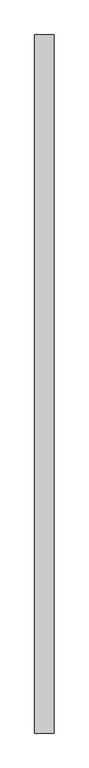
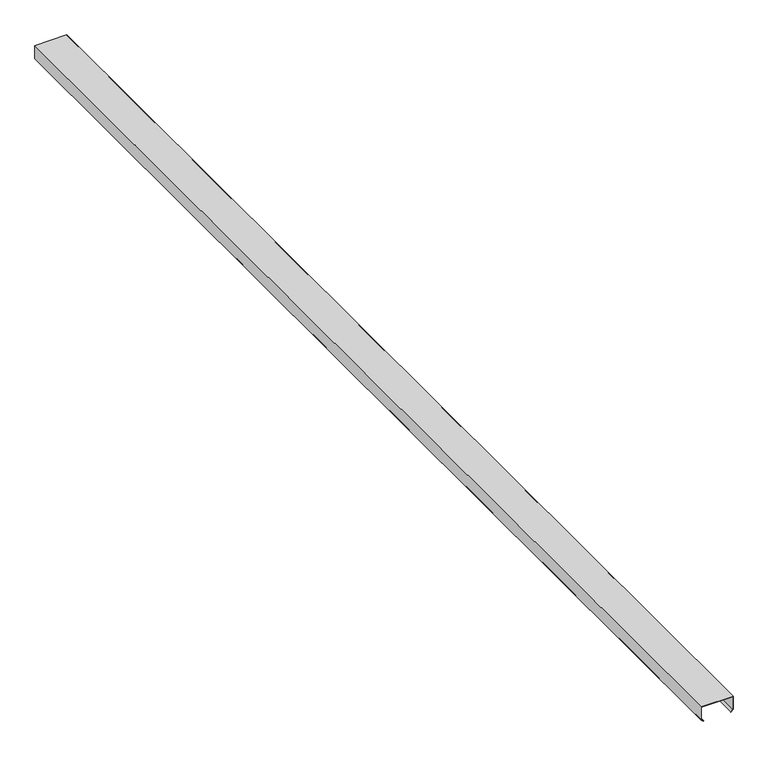
"""IFC4 building model written with IfcOpenShell, lengths in millimetres: proxy geometry, Generic Models 7:Generic Models 1:1:Generic Models 1:1 : Generic Models 7:Generic Models 1:337419:19 : Generic Models 7:Generic Models 1:1:Generic Models 1:1 : Generic Models 7:Generic Models 1:337419:306201."""

import ifcopenshell
import ifcopenshell.guid

model = None  # the IFC model being written
_history = None  # IfcOwnerHistory: only IFC2X3 demands one
_inside = {}  # id of a spatial element -> (the spatial element, [elements in it])
_under = {}  # id of a project, library or spatial element -> (it, [spatial elements below it])
_declared = {}  # id of a project -> (the project, [libraries it declares])
_typed = {}  # id of a type object -> (the type object, [elements of that type])
_made_of = {}  # id of a material, layer set ... -> (it, [elements and type objects made of it])


def new_model(schema):
    """Start an empty IFC model of exactly this schema.

    Asked for "IFC4X3", IfcOpenShell would pick the latest addendum, in which some entities
    have other attributes; the version numbers below select the first issue.
    IFC2X3 requires an IfcOwnerHistory on every rooted entity: one is made here for all.
    """
    global model, _history
    if schema == "IFC4X3":
        model = ifcopenshell.file(schema_version=(4, 3, 0, 0))
    else:
        model = ifcopenshell.file(schema=schema)
    _inside.clear()
    _under.clear()
    _declared.clear()
    _typed.clear()
    _made_of.clear()
    _history = None
    if model.schema == "IFC2X3":
        org = make("IfcOrganization", Name="unknown")
        user = make(
            "IfcPersonAndOrganization",
            ThePerson=make("IfcPerson", FamilyName="unknown"),
            TheOrganization=org,
        )
        app = make(
            "IfcApplication",
            ApplicationDeveloper=org,
            Version="unknown",
            ApplicationFullName="unknown",
            ApplicationIdentifier="unknown",
        )
        _history = make(
            "IfcOwnerHistory",
            OwningUser=user,
            OwningApplication=app,
            ChangeAction="ADDED",
            CreationDate=0,
        )
    return model


def make(cls, **values):
    """One entity of the class cls with the attributes given. An attribute that is None is left unset."""
    return model.create_entity(
        cls, **{name: value for name, value in values.items() if value is not None}
    )


def rooted(cls, **values):
    """An entity with a GlobalId (a new one), such as an element, a storey or a relation."""
    return make(cls, GlobalId=ifcopenshell.guid.new(), OwnerHistory=_history, **values)


def si_unit(unit_type, name, prefix=None):
    """IfcSIUnit, for example si_unit("LENGTHUNIT", "METRE", prefix="MILLI")."""
    return make("IfcSIUnit", UnitType=unit_type, Prefix=prefix, Name=name)


def assignment(units):
    """IfcUnitAssignment: the units of a project."""
    return None if units is None else make("IfcUnitAssignment", Units=units)


def point(xyz):
    """IfcCartesianPoint."""
    return None if xyz is None else make("IfcCartesianPoint", Coordinates=xyz)


def direction(xyz):
    """IfcDirection."""
    return None if xyz is None else make("IfcDirection", DirectionRatios=xyz)


def frame(location, z_axis=None, x_axis=None):
    """IfcAxis2Placement3D, a coordinate frame: its origin and axes. An axis left out is left unset."""
    return make(
        "IfcAxis2Placement3D",
        Location=point(location),
        Axis=direction(z_axis),
        RefDirection=direction(x_axis),
    )


def origin():
    """The frame at (0, 0, 0) with its axes left unset."""
    return frame((0.0, 0.0, 0.0))


def place(relative_to, where):
    """IfcLocalPlacement: puts the frame where relative to a parent placement (None: the world)."""
    return make(
        "IfcLocalPlacement", PlacementRelTo=relative_to, RelativePlacement=where
    )


def context(
    kind, dimensions, precision=None, world=None, true_north=None, identifier=None
):
    """IfcGeometricRepresentationContext, for example the 3D "Model" context."""
    return make(
        "IfcGeometricRepresentationContext",
        ContextIdentifier=identifier,
        ContextType=kind,
        CoordinateSpaceDimension=dimensions,
        Precision=precision,
        WorldCoordinateSystem=world,
        TrueNorth=true_north,
    )


def project(units=None, contexts=None):
    """IfcProject with its units and contexts."""
    return rooted(
        "IfcProject",
        Name="project",
        RepresentationContexts=contexts,
        UnitsInContext=assignment(units),
    )


def spatial(cls, under=None, at=None, **own):
    """A site, building, storey or space (cls), placed at a placement, below another one or the project."""
    s = rooted(cls, ObjectPlacement=at, **own)
    if under is not None:
        _under.setdefault(under.id(), (under, []))[1].append(s)
    return s


def polyline(points):
    """IfcPolyline through the points."""
    return make("IfcPolyline", Points=[point(p) for p in points])


def outline(outer, holes=None, kind="AREA"):
    """IfcArbitraryClosedProfileDef: a profile drawn as a closed curve; with holes, ...WithVoids."""
    if holes is None:
        return make("IfcArbitraryClosedProfileDef", ProfileType=kind, OuterCurve=outer)
    return make(
        "IfcArbitraryProfileDefWithVoids",
        ProfileType=kind,
        OuterCurve=outer,
        InnerCurves=holes,
    )


def extrude(swept, where, along, depth):
    """IfcExtrudedAreaSolid: the profile swept, set in the frame where, extruded along a direction by depth."""
    return make(
        "IfcExtrudedAreaSolid",
        SweptArea=swept,
        Position=where,
        ExtrudedDirection=direction(along),
        Depth=depth,
    )


def shape(context_of_items, identifier, shape_type, items):
    """IfcShapeRepresentation: the items that make up one representation, for example the "Body"."""
    return make(
        "IfcShapeRepresentation",
        ContextOfItems=context_of_items,
        RepresentationIdentifier=identifier,
        RepresentationType=shape_type,
        Items=items,
    )


def source(mapping_origin, context_of_items, identifier, shape_type, items):
    """IfcRepresentationMap: a shape defined once, which mapped items show again and again."""
    return make(
        "IfcRepresentationMap",
        MappingOrigin=mapping_origin,
        MappedRepresentation=shape(context_of_items, identifier, shape_type, items),
    )


def transform(
    local_origin,
    x_axis=None,
    y_axis=None,
    z_axis=None,
    scale=None,
    scale2=None,
    scale3=None,
    uniform=True,
):
    """IfcCartesianTransformationOperator3D, or its non-uniform kind. x_axis, y_axis, z_axis: its Axis1, 2, 3."""
    if uniform:
        return make(
            "IfcCartesianTransformationOperator3D",
            Axis1=direction(x_axis),
            Axis2=direction(y_axis),
            LocalOrigin=point(local_origin),
            Scale=scale,
            Axis3=direction(z_axis),
        )
    return make(
        "IfcCartesianTransformationOperator3DnonUniform",
        Axis1=direction(x_axis),
        Axis2=direction(y_axis),
        LocalOrigin=point(local_origin),
        Scale=scale,
        Axis3=direction(z_axis),
        Scale2=scale2,
        Scale3=scale3,
    )


def mapped(mapping_source, mapping_target):
    """IfcMappedItem: shows the shape of a source again, moved by a transform."""
    return make(
        "IfcMappedItem", MappingSource=mapping_source, MappingTarget=mapping_target
    )


def made_of(thing, what):
    """Note that an element or type object is made of a material, layer set ...; save() writes the relation."""
    if what is not None:
        _made_of.setdefault(what.id(), (what, []))[1].append(thing)
    return thing


def element(
    cls,
    number,
    at=None,
    inside=None,
    cuts=None,
    type_object=None,
    material=None,
    context=None,
    identifier="Body",
    shape_type=None,
    held_by="IfcProductDefinitionShape",
    body=None,
    shapes=None,
    **own,
):
    """One element of the class cls, such as IfcWall. Its Tag is "e" and its number.

    at: its placement. inside: the storey or other place that contains it. cuts: it is an
    opening in that element (IfcRelVoidsElement). A single representation is given by context,
    identifier, shape_type and body (its items); several are given by shapes. held_by: the class
    of the entity that holds the representations. save() writes the other relations.
    """
    e = rooted(cls, Tag="e%d" % number, ObjectPlacement=at, **own)
    if body is not None:
        shapes = [shape(context, identifier, shape_type, body)]
    if shapes is not None:
        e.Representation = make(held_by, Representations=shapes)
    if inside is not None:
        _inside.setdefault(inside.id(), (inside, []))[1].append(e)
    if cuts is not None:
        rooted(
            "IfcRelVoidsElement", RelatingBuildingElement=cuts, RelatedOpeningElement=e
        )
    if type_object is not None:
        _typed.setdefault(type_object.id(), (type_object, []))[1].append(e)
    return made_of(e, material)


def aggregate(whole, parts):
    """IfcRelAggregates: a whole, such as a stair, and the parts it consists of."""
    return rooted("IfcRelAggregates", RelatingObject=whole, RelatedObjects=parts)


def save(model, path):
    """Write the relations noted so far, then the file.

    IfcRelAggregates (storeys below a building ...), IfcRelContainedInSpatialStructure (elements
    in a storey), IfcRelDefinesByType, IfcRelAssociatesMaterial and IfcRelDeclares: one each for
    every whole, place, type object, material and project.
    """
    for whole, parts in _under.values():
        aggregate(whole, parts)
    for where, things in _inside.values():
        rooted(
            "IfcRelContainedInSpatialStructure",
            RelatedElements=things,
            RelatingStructure=where,
        )
    for kind, things in _typed.values():
        rooted("IfcRelDefinesByType", RelatedObjects=things, RelatingType=kind)
    for what, things in _made_of.values():
        rooted("IfcRelAssociatesMaterial", RelatedObjects=things, RelatingMaterial=what)
    for by, libraries in _declared.values():
        rooted("IfcRelDeclares", RelatingContext=by, RelatedDefinitions=libraries)
    model.write(path)


def generic_models_2c2944e3(model_context):
    return source(origin(), model_context, "Body", "SweptSolid", [
        extrude(outline(polyline([(6128.940625, 579307.711724), (6128.940625, 579104.511724), (6040.040625, 579104.511724), (6027.7955211, 579119.1048707), (6029.9236883, 579120.890615), (6041.336086, 579107.289849), (6126.1625, 579107.289849), (6126.1625, 579304.933599), (6041.336086, 579304.933599), (6029.9236883, 579291.3328331), (6027.7955211, 579293.1185774), (6040.040625, 579307.711724), (6128.940625, 579307.711724)])), frame((0.0, -581258.1163841, 0.0), z_axis=(0.0, 1.0, 0.0), x_axis=(0.0, 0.0, 1.0)), (0.0, 0.0, 1.0), 7315.2),
    ])


if __name__ == "__main__":
    model = new_model("IFC4")
    model_context = context("Model", 3, world=origin())
    ifc_project = project(units=[si_unit("LENGTHUNIT", "METRE", prefix="MILLI")], contexts=[model_context])
    site = spatial("IfcSite", under=ifc_project)
    building = spatial("IfcBuilding", under=site)
    placement = place(None, origin())
    generic_models_shape = generic_models_2c2944e3(model_context)
    element("IfcBuildingElementProxy", 1, Name="Generic Models 7:Generic Models 1:1:Generic Models 1:1 : Generic Models 7:Generic Models 1:337419:19 : Generic Models 7:Generic Models 1:1:Generic Models 1:1 : Generic Models 7:Generic Models 1:337419:306201", ObjectType="Generic Models 7:Generic Models 1:1:Generic Models 1:1 : Generic Models 7:Generic Models 1:337419:19 : Generic Models 7:Generic Models 1:1:Generic Models 1:1 : Generic Models 7:Generic Models 1:337419:306201", at=placement, inside=building, context=model_context, shape_type="MappedRepresentation", body=[
        mapped(generic_models_shape, transform((0.0, 0.0, 0.0), x_axis=(1.0, 0.0, 0.0), y_axis=(0.0, 1.0, 0.0), z_axis=(0.0, 0.0, 1.0))),
    ])
    save(model, "model.ifc")

# Revit data of these elements
# Type "Generic Models 7:Generic Models 1:1:Generic Models 1:1 : Generic Models 7:Generic Models 1:337419:19 : Generic Models 7:Generic Models 1:1:Generic Models 1:1 : Generic Models 7:Generic Models 1:337419:306201"
#   NameOverride = "Generic Models 7:Generic Models 1:1:Generic Models 1:1 : Generic Models 7:Generic Models 1:337419:306201"
#   ObjectTypeOverride = "Generic Models 1:1 : Generic Models 7:Generic Models 1:337419"
#   Reference = "Generic Models 1"
#   Tag = "306201"
# Element 1 (IfcBuildingElementProxy, "Generic Models 7:Generic Models 1:1:Generic Models 1:1 : Generic Models 7:Generic Models 1:337419:19 : Generic Models 7:Generic Models 1:1:Generic Models 1:1 : Generic Models 7:Generic Models 1:337419:306201")
#   Materials on its faces: "'ZEE' SECTION (8.0x3.5Z - SEE STRUCT. DWGS)"
# Materials
#   "'ZEE' SECTION (8.0x3.5Z - SEE STRUCT. DWGS)": class "Unassigned", colour RGB 210 209 208, transparency 0, Keynote = "M05121300.02", Cost = 0
